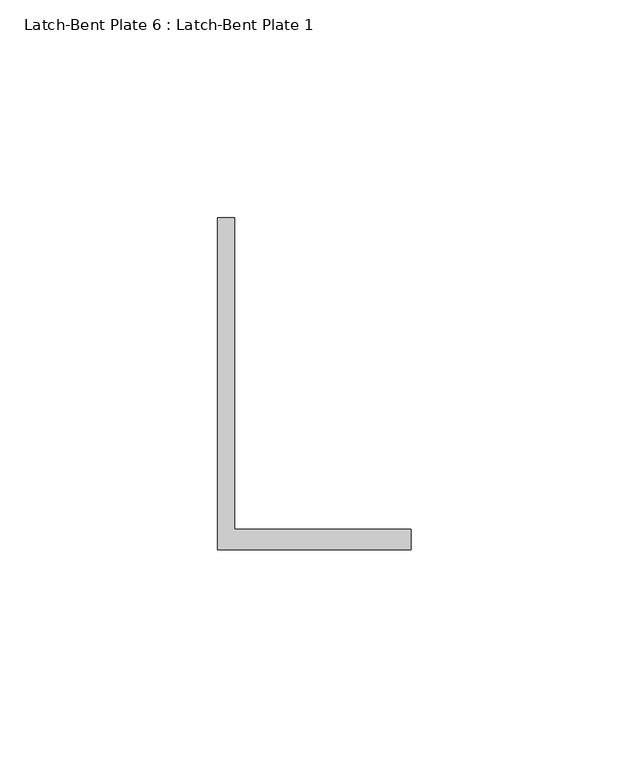
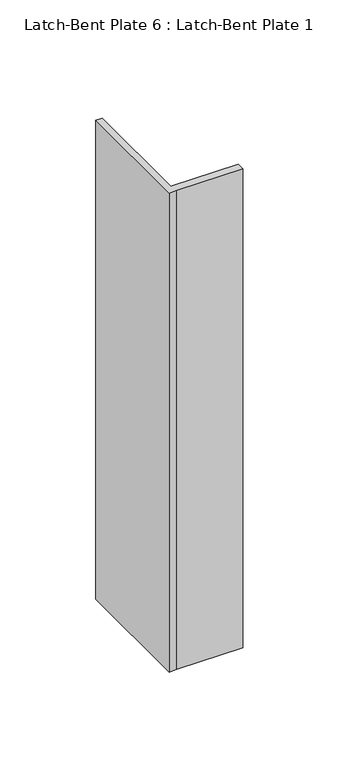
"""IFC4 building model written with IfcOpenShell, lengths in millimetres: proxy geometry, Latch-Bent Plate 6 : Latch-Bent Plate 1."""

import ifcopenshell
import ifcopenshell.guid

model = None  # the IFC model being written
_history = None  # IfcOwnerHistory: only IFC2X3 demands one
_inside = {}  # id of a spatial element -> (the spatial element, [elements in it])
_under = {}  # id of a project, library or spatial element -> (it, [spatial elements below it])
_declared = {}  # id of a project -> (the project, [libraries it declares])
_typed = {}  # id of a type object -> (the type object, [elements of that type])
_made_of = {}  # id of a material, layer set ... -> (it, [elements and type objects made of it])


def new_model(schema):
    """Start an empty IFC model of exactly this schema.

    Asked for "IFC4X3", IfcOpenShell would pick the latest addendum, in which some entities
    have other attributes; the version numbers below select the first issue.
    IFC2X3 requires an IfcOwnerHistory on every rooted entity: one is made here for all.
    """
    global model, _history
    if schema == "IFC4X3":
        model = ifcopenshell.file(schema_version=(4, 3, 0, 0))
    else:
        model = ifcopenshell.file(schema=schema)
    _inside.clear()
    _under.clear()
    _declared.clear()
    _typed.clear()
    _made_of.clear()
    _history = None
    if model.schema == "IFC2X3":
        org = make("IfcOrganization", Name="unknown")
        user = make(
            "IfcPersonAndOrganization",
            ThePerson=make("IfcPerson", FamilyName="unknown"),
            TheOrganization=org,
        )
        app = make(
            "IfcApplication",
            ApplicationDeveloper=org,
            Version="unknown",
            ApplicationFullName="unknown",
            ApplicationIdentifier="unknown",
        )
        _history = make(
            "IfcOwnerHistory",
            OwningUser=user,
            OwningApplication=app,
            ChangeAction="ADDED",
            CreationDate=0,
        )
    return model


def make(cls, **values):
    """One entity of the class cls with the attributes given. An attribute that is None is left unset."""
    return model.create_entity(
        cls, **{name: value for name, value in values.items() if value is not None}
    )


def rooted(cls, **values):
    """An entity with a GlobalId (a new one), such as an element, a storey or a relation."""
    return make(cls, GlobalId=ifcopenshell.guid.new(), OwnerHistory=_history, **values)


def si_unit(unit_type, name, prefix=None):
    """IfcSIUnit, for example si_unit("LENGTHUNIT", "METRE", prefix="MILLI")."""
    return make("IfcSIUnit", UnitType=unit_type, Prefix=prefix, Name=name)


def assignment(units):
    """IfcUnitAssignment: the units of a project."""
    return None if units is None else make("IfcUnitAssignment", Units=units)


def point(xyz):
    """IfcCartesianPoint."""
    return None if xyz is None else make("IfcCartesianPoint", Coordinates=xyz)


def direction(xyz):
    """IfcDirection."""
    return None if xyz is None else make("IfcDirection", DirectionRatios=xyz)


def frame(location, z_axis=None, x_axis=None):
    """IfcAxis2Placement3D, a coordinate frame: its origin and axes. An axis left out is left unset."""
    return make(
        "IfcAxis2Placement3D",
        Location=point(location),
        Axis=direction(z_axis),
        RefDirection=direction(x_axis),
    )


def origin():
    """The frame at (0, 0, 0) with its axes left unset."""
    return frame((0.0, 0.0, 0.0))


def place(relative_to, where):
    """IfcLocalPlacement: puts the frame where relative to a parent placement (None: the world)."""
    return make(
        "IfcLocalPlacement", PlacementRelTo=relative_to, RelativePlacement=where
    )


def context(
    kind, dimensions, precision=None, world=None, true_north=None, identifier=None
):
    """IfcGeometricRepresentationContext, for example the 3D "Model" context."""
    return make(
        "IfcGeometricRepresentationContext",
        ContextIdentifier=identifier,
        ContextType=kind,
        CoordinateSpaceDimension=dimensions,
        Precision=precision,
        WorldCoordinateSystem=world,
        TrueNorth=true_north,
    )


def project(units=None, contexts=None):
    """IfcProject with its units and contexts."""
    return rooted(
        "IfcProject",
        Name="project",
        RepresentationContexts=contexts,
        UnitsInContext=assignment(units),
    )


def spatial(cls, under=None, at=None, **own):
    """A site, building, storey or space (cls), placed at a placement, below another one or the project."""
    s = rooted(cls, ObjectPlacement=at, **own)
    if under is not None:
        _under.setdefault(under.id(), (under, []))[1].append(s)
    return s


def polyline(points):
    """IfcPolyline through the points."""
    return make("IfcPolyline", Points=[point(p) for p in points])


def outline(outer, holes=None, kind="AREA"):
    """IfcArbitraryClosedProfileDef: a profile drawn as a closed curve; with holes, ...WithVoids."""
    if holes is None:
        return make("IfcArbitraryClosedProfileDef", ProfileType=kind, OuterCurve=outer)
    return make(
        "IfcArbitraryProfileDefWithVoids",
        ProfileType=kind,
        OuterCurve=outer,
        InnerCurves=holes,
    )


def extrude(swept, where, along, depth):
    """IfcExtrudedAreaSolid: the profile swept, set in the frame where, extruded along a direction by depth."""
    return make(
        "IfcExtrudedAreaSolid",
        SweptArea=swept,
        Position=where,
        ExtrudedDirection=direction(along),
        Depth=depth,
    )


def shape(context_of_items, identifier, shape_type, items):
    """IfcShapeRepresentation: the items that make up one representation, for example the "Body"."""
    return make(
        "IfcShapeRepresentation",
        ContextOfItems=context_of_items,
        RepresentationIdentifier=identifier,
        RepresentationType=shape_type,
        Items=items,
    )


def source(mapping_origin, context_of_items, identifier, shape_type, items):
    """IfcRepresentationMap: a shape defined once, which mapped items show again and again."""
    return make(
        "IfcRepresentationMap",
        MappingOrigin=mapping_origin,
        MappedRepresentation=shape(context_of_items, identifier, shape_type, items),
    )


def transform(
    local_origin,
    x_axis=None,
    y_axis=None,
    z_axis=None,
    scale=None,
    scale2=None,
    scale3=None,
    uniform=True,
):
    """IfcCartesianTransformationOperator3D, or its non-uniform kind. x_axis, y_axis, z_axis: its Axis1, 2, 3."""
    if uniform:
        return make(
            "IfcCartesianTransformationOperator3D",
            Axis1=direction(x_axis),
            Axis2=direction(y_axis),
            LocalOrigin=point(local_origin),
            Scale=scale,
            Axis3=direction(z_axis),
        )
    return make(
        "IfcCartesianTransformationOperator3DnonUniform",
        Axis1=direction(x_axis),
        Axis2=direction(y_axis),
        LocalOrigin=point(local_origin),
        Scale=scale,
        Axis3=direction(z_axis),
        Scale2=scale2,
        Scale3=scale3,
    )


def mapped(mapping_source, mapping_target):
    """IfcMappedItem: shows the shape of a source again, moved by a transform."""
    return make(
        "IfcMappedItem", MappingSource=mapping_source, MappingTarget=mapping_target
    )


def made_of(thing, what):
    """Note that an element or type object is made of a material, layer set ...; save() writes the relation."""
    if what is not None:
        _made_of.setdefault(what.id(), (what, []))[1].append(thing)
    return thing


def element(
    cls,
    number,
    at=None,
    inside=None,
    cuts=None,
    type_object=None,
    material=None,
    context=None,
    identifier="Body",
    shape_type=None,
    held_by="IfcProductDefinitionShape",
    body=None,
    shapes=None,
    **own,
):
    """One element of the class cls, such as IfcWall. Its Tag is "e" and its number.

    at: its placement. inside: the storey or other place that contains it. cuts: it is an
    opening in that element (IfcRelVoidsElement). A single representation is given by context,
    identifier, shape_type and body (its items); several are given by shapes. held_by: the class
    of the entity that holds the representations. save() writes the other relations.
    """
    e = rooted(cls, Tag="e%d" % number, ObjectPlacement=at, **own)
    if body is not None:
        shapes = [shape(context, identifier, shape_type, body)]
    if shapes is not None:
        e.Representation = make(held_by, Representations=shapes)
    if inside is not None:
        _inside.setdefault(inside.id(), (inside, []))[1].append(e)
    if cuts is not None:
        rooted(
            "IfcRelVoidsElement", RelatingBuildingElement=cuts, RelatedOpeningElement=e
        )
    if type_object is not None:
        _typed.setdefault(type_object.id(), (type_object, []))[1].append(e)
    return made_of(e, material)


def aggregate(whole, parts):
    """IfcRelAggregates: a whole, such as a stair, and the parts it consists of."""
    return rooted("IfcRelAggregates", RelatingObject=whole, RelatedObjects=parts)


def save(model, path):
    """Write the relations noted so far, then the file.

    IfcRelAggregates (storeys below a building ...), IfcRelContainedInSpatialStructure (elements
    in a storey), IfcRelDefinesByType, IfcRelAssociatesMaterial and IfcRelDeclares: one each for
    every whole, place, type object, material and project.
    """
    for whole, parts in _under.values():
        aggregate(whole, parts)
    for where, things in _inside.values():
        rooted(
            "IfcRelContainedInSpatialStructure",
            RelatedElements=things,
            RelatingStructure=where,
        )
    for kind, things in _typed.values():
        rooted("IfcRelDefinesByType", RelatedObjects=things, RelatingType=kind)
    for what, things in _made_of.values():
        rooted("IfcRelAssociatesMaterial", RelatedObjects=things, RelatingMaterial=what)
    for by, libraries in _declared.values():
        rooted("IfcRelDeclares", RelatingContext=by, RelatedDefinitions=libraries)
    model.write(path)


def latch_bent_plate_6_latch_bent_plate_1_8bdba4d9(model_context):
    return source(origin(), model_context, "Body", "SweptSolid", [
        extrude(outline(polyline([(587327.0060739, -535201.5663841), (587322.2435739, -535201.5663841), (587322.2435739, -535125.3663841), (587326.1141748, -535125.3663841), (587326.1141748, -535196.8038841), (587366.6808739, -535196.8038841), (587366.6808739, -535201.5663841), (587327.0060739, -535201.5663841)])), frame((0.0, 0.0, 50.8), z_axis=(0.0, 0.0, 1.0), x_axis=(1.0, 0.0, 0.0)), (0.0, 0.0, 1.0), 304.8),
    ])


if __name__ == "__main__":
    model = new_model("IFC4")
    model_context = context("Model", 3, world=origin())
    ifc_project = project(units=[si_unit("LENGTHUNIT", "METRE", prefix="MILLI")], contexts=[model_context])
    site = spatial("IfcSite", under=ifc_project)
    building = spatial("IfcBuilding", under=site)
    placement = place(None, origin())
    latch_bent_plate_6_latch_bent_plate_1_shape = latch_bent_plate_6_latch_bent_plate_1_8bdba4d9(model_context)
    element("IfcBuildingElementProxy", 1, Name="Latch-Bent Plate 6 : Latch-Bent Plate 1", ObjectType="Latch-Bent Plate 6 : Latch-Bent Plate 1", at=placement, inside=building, context=model_context, shape_type="MappedRepresentation", body=[
        mapped(latch_bent_plate_6_latch_bent_plate_1_shape, transform((0.0, 0.0, 0.0), x_axis=(1.0, 0.0, 0.0), y_axis=(0.0, 1.0, 0.0), z_axis=(0.0, 0.0, 1.0))),
    ])
    save(model, "model.ifc")

# Revit data of these elements
# Element 1 (IfcBuildingElementProxy, "Latch-Bent Plate 6 : Latch-Bent Plate 1")
#   Materials on its faces: "GALV. GATE LATCH"
# Materials
#   "GALV. GATE LATCH": class "Metal", colour RGB 189 187 185, transparency 0, Description = "Carbon steel", Cost = 0
